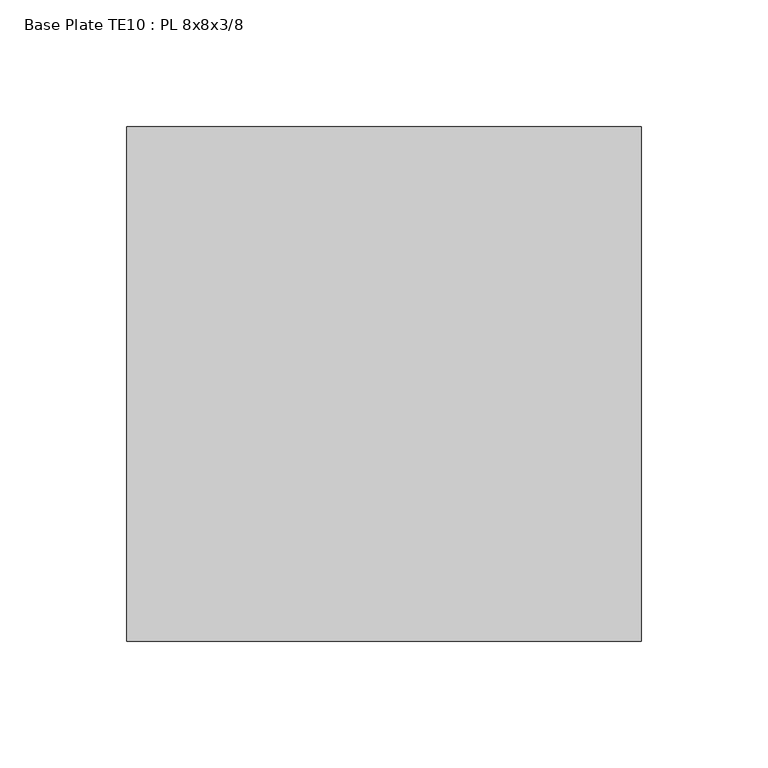
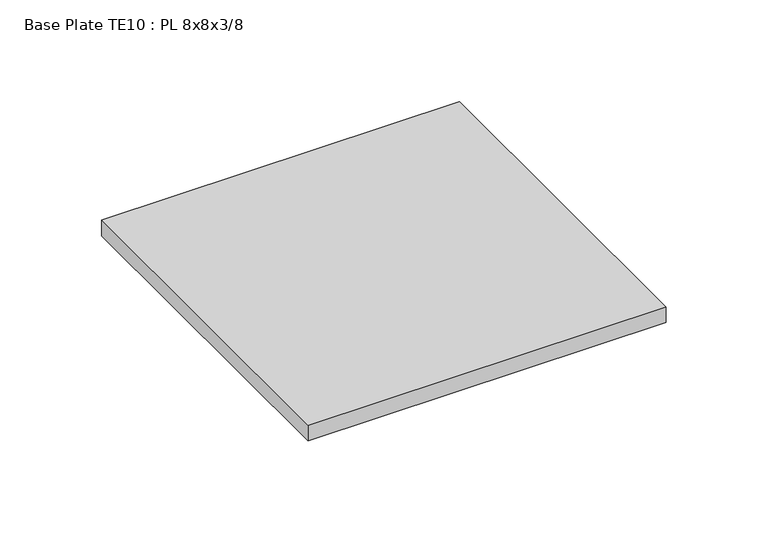
"""IFC4 building model written with IfcOpenShell, lengths in millimetres: proxy geometry, Base Plate TE10 : PL 8x8x3/8."""

from ifc_helpers import new_model, si_unit, frame, origin, place, context, project, spatial, polyline, outline, extrude, source, transform, mapped, element, save


def base_plate_te10_pl_8x8x3_8_a06680a7(model_context):
    return source(origin(), model_context, "Body", "SweptSolid", [
        extrude(outline(polyline([(590318.6599233, -532779.0413841), (590318.6599233, -532982.2413841), (590115.4599233, -532982.2413841), (590115.4599233, -532779.0413841), (590318.6599233, -532779.0413841)])), frame((0.0, 0.0, 19.05), z_axis=(0.0, 0.0, 1.0), x_axis=(1.0, 0.0, 0.0)), (0.0, 0.0, 1.0), 9.525),
    ])


if __name__ == "__main__":
    model = new_model("IFC4")
    model_context = context("Model", 3, world=origin())
    ifc_project = project(units=[si_unit("LENGTHUNIT", "METRE", prefix="MILLI")], contexts=[model_context])
    site = spatial("IfcSite", under=ifc_project)
    building = spatial("IfcBuilding", under=site)
    placement = place(None, origin())
    base_plate_te10_pl_8x8x3_8_shape = base_plate_te10_pl_8x8x3_8_a06680a7(model_context)
    element("IfcBuildingElementProxy", 1, Name="Base Plate TE10 : PL 8x8x3/8", ObjectType="Base Plate TE10 : PL 8x8x3/8", at=placement, inside=building, context=model_context, shape_type="MappedRepresentation", body=[
        mapped(base_plate_te10_pl_8x8x3_8_shape, transform((0.0, 0.0, 0.0), x_axis=(1.0, 0.0, 0.0), y_axis=(0.0, 1.0, 0.0), z_axis=(0.0, 0.0, 1.0))),
    ])
    save(model, "model.ifc")

# Revit data of these elements
# Element 1 (IfcBuildingElementProxy, "Base Plate TE10 : PL 8x8x3/8")
#   Materials on its faces: "GALV. STL BASE PLATE"
# Materials
#   "GALV. STL BASE PLATE": class "Generic", colour RGB 211 211 207, transparency 0, Cost = 0
